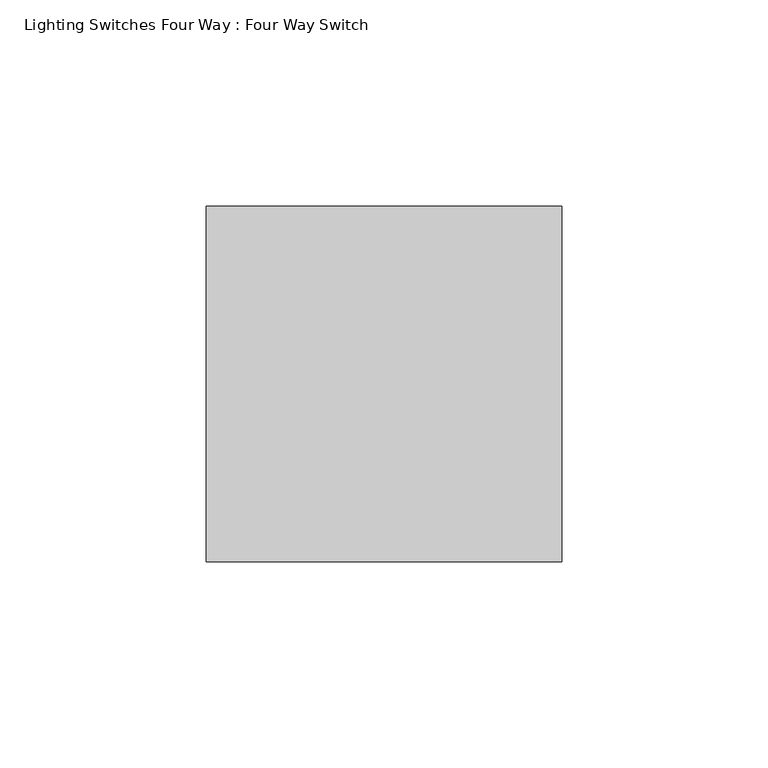
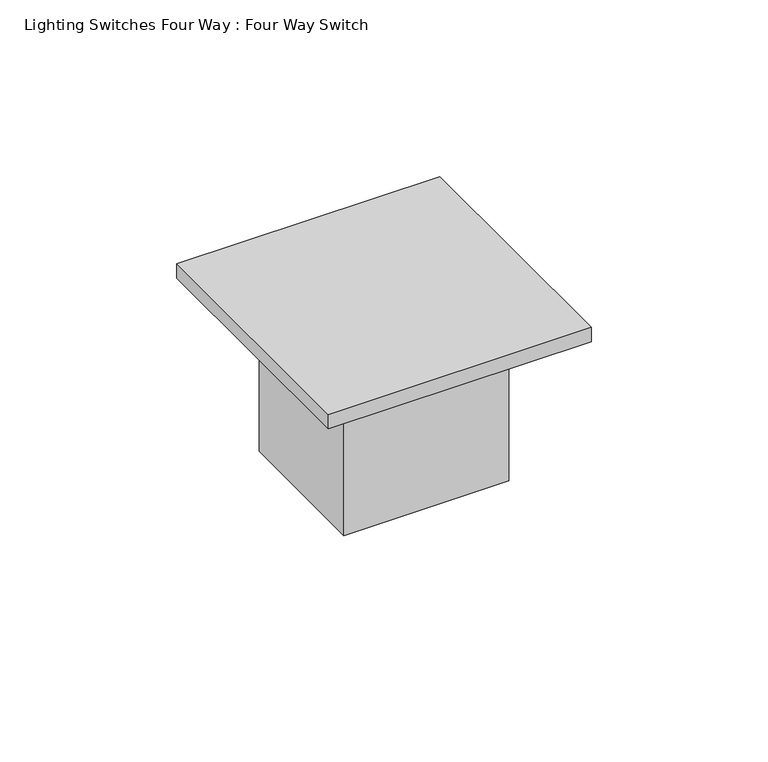
"""IFC4 building model written with IfcOpenShell, lengths in millimetres: switching device geometry, Lighting Switches Four Way : Four Way Switch."""

import ifcopenshell
import ifcopenshell.guid

model = None  # the IFC model being written
_history = None  # IfcOwnerHistory: only IFC2X3 demands one
_inside = {}  # id of a spatial element -> (the spatial element, [elements in it])
_under = {}  # id of a project, library or spatial element -> (it, [spatial elements below it])
_declared = {}  # id of a project -> (the project, [libraries it declares])
_typed = {}  # id of a type object -> (the type object, [elements of that type])
_made_of = {}  # id of a material, layer set ... -> (it, [elements and type objects made of it])


def new_model(schema):
    """Start an empty IFC model of exactly this schema.

    Asked for "IFC4X3", IfcOpenShell would pick the latest addendum, in which some entities
    have other attributes; the version numbers below select the first issue.
    IFC2X3 requires an IfcOwnerHistory on every rooted entity: one is made here for all.
    """
    global model, _history
    if schema == "IFC4X3":
        model = ifcopenshell.file(schema_version=(4, 3, 0, 0))
    else:
        model = ifcopenshell.file(schema=schema)
    _inside.clear()
    _under.clear()
    _declared.clear()
    _typed.clear()
    _made_of.clear()
    _history = None
    if model.schema == "IFC2X3":
        org = make("IfcOrganization", Name="unknown")
        user = make(
            "IfcPersonAndOrganization",
            ThePerson=make("IfcPerson", FamilyName="unknown"),
            TheOrganization=org,
        )
        app = make(
            "IfcApplication",
            ApplicationDeveloper=org,
            Version="unknown",
            ApplicationFullName="unknown",
            ApplicationIdentifier="unknown",
        )
        _history = make(
            "IfcOwnerHistory",
            OwningUser=user,
            OwningApplication=app,
            ChangeAction="ADDED",
            CreationDate=0,
        )
    return model


def make(cls, **values):
    """One entity of the class cls with the attributes given. An attribute that is None is left unset."""
    return model.create_entity(
        cls, **{name: value for name, value in values.items() if value is not None}
    )


def rooted(cls, **values):
    """An entity with a GlobalId (a new one), such as an element, a storey or a relation."""
    return make(cls, GlobalId=ifcopenshell.guid.new(), OwnerHistory=_history, **values)


def si_unit(unit_type, name, prefix=None):
    """IfcSIUnit, for example si_unit("LENGTHUNIT", "METRE", prefix="MILLI")."""
    return make("IfcSIUnit", UnitType=unit_type, Prefix=prefix, Name=name)


def assignment(units):
    """IfcUnitAssignment: the units of a project."""
    return None if units is None else make("IfcUnitAssignment", Units=units)


def point(xyz):
    """IfcCartesianPoint."""
    return None if xyz is None else make("IfcCartesianPoint", Coordinates=xyz)


def direction(xyz):
    """IfcDirection."""
    return None if xyz is None else make("IfcDirection", DirectionRatios=xyz)


def frame(location, z_axis=None, x_axis=None):
    """IfcAxis2Placement3D, a coordinate frame: its origin and axes. An axis left out is left unset."""
    return make(
        "IfcAxis2Placement3D",
        Location=point(location),
        Axis=direction(z_axis),
        RefDirection=direction(x_axis),
    )


def origin():
    """The frame at (0, 0, 0) with its axes left unset."""
    return frame((0.0, 0.0, 0.0))


def origin_with_axes():
    """The frame at (0, 0, 0) with the z axis (0, 0, 1) and the x axis (1, 0, 0) written out."""
    return frame((0.0, 0.0, 0.0), z_axis=(0.0, 0.0, 1.0), x_axis=(1.0, 0.0, 0.0))


def place(relative_to, where):
    """IfcLocalPlacement: puts the frame where relative to a parent placement (None: the world)."""
    return make(
        "IfcLocalPlacement", PlacementRelTo=relative_to, RelativePlacement=where
    )


def context(
    kind, dimensions, precision=None, world=None, true_north=None, identifier=None
):
    """IfcGeometricRepresentationContext, for example the 3D "Model" context."""
    return make(
        "IfcGeometricRepresentationContext",
        ContextIdentifier=identifier,
        ContextType=kind,
        CoordinateSpaceDimension=dimensions,
        Precision=precision,
        WorldCoordinateSystem=world,
        TrueNorth=true_north,
    )


def project(units=None, contexts=None):
    """IfcProject with its units and contexts."""
    return rooted(
        "IfcProject",
        Name="project",
        RepresentationContexts=contexts,
        UnitsInContext=assignment(units),
    )


def spatial(cls, under=None, at=None, **own):
    """A site, building, storey or space (cls), placed at a placement, below another one or the project."""
    s = rooted(cls, ObjectPlacement=at, **own)
    if under is not None:
        _under.setdefault(under.id(), (under, []))[1].append(s)
    return s


def polyline(points):
    """IfcPolyline through the points."""
    return make("IfcPolyline", Points=[point(p) for p in points])


def outline(outer, holes=None, kind="AREA"):
    """IfcArbitraryClosedProfileDef: a profile drawn as a closed curve; with holes, ...WithVoids."""
    if holes is None:
        return make("IfcArbitraryClosedProfileDef", ProfileType=kind, OuterCurve=outer)
    return make(
        "IfcArbitraryProfileDefWithVoids",
        ProfileType=kind,
        OuterCurve=outer,
        InnerCurves=holes,
    )


def extrude(swept, where, along, depth):
    """IfcExtrudedAreaSolid: the profile swept, set in the frame where, extruded along a direction by depth."""
    return make(
        "IfcExtrudedAreaSolid",
        SweptArea=swept,
        Position=where,
        ExtrudedDirection=direction(along),
        Depth=depth,
    )


def shape(context_of_items, identifier, shape_type, items):
    """IfcShapeRepresentation: the items that make up one representation, for example the "Body"."""
    return make(
        "IfcShapeRepresentation",
        ContextOfItems=context_of_items,
        RepresentationIdentifier=identifier,
        RepresentationType=shape_type,
        Items=items,
    )


def source(mapping_origin, context_of_items, identifier, shape_type, items):
    """IfcRepresentationMap: a shape defined once, which mapped items show again and again."""
    return make(
        "IfcRepresentationMap",
        MappingOrigin=mapping_origin,
        MappedRepresentation=shape(context_of_items, identifier, shape_type, items),
    )


def transform(
    local_origin,
    x_axis=None,
    y_axis=None,
    z_axis=None,
    scale=None,
    scale2=None,
    scale3=None,
    uniform=True,
):
    """IfcCartesianTransformationOperator3D, or its non-uniform kind. x_axis, y_axis, z_axis: its Axis1, 2, 3."""
    if uniform:
        return make(
            "IfcCartesianTransformationOperator3D",
            Axis1=direction(x_axis),
            Axis2=direction(y_axis),
            LocalOrigin=point(local_origin),
            Scale=scale,
            Axis3=direction(z_axis),
        )
    return make(
        "IfcCartesianTransformationOperator3DnonUniform",
        Axis1=direction(x_axis),
        Axis2=direction(y_axis),
        LocalOrigin=point(local_origin),
        Scale=scale,
        Axis3=direction(z_axis),
        Scale2=scale2,
        Scale3=scale3,
    )


def mapped(mapping_source, mapping_target):
    """IfcMappedItem: shows the shape of a source again, moved by a transform."""
    return make(
        "IfcMappedItem", MappingSource=mapping_source, MappingTarget=mapping_target
    )


def made_of(thing, what):
    """Note that an element or type object is made of a material, layer set ...; save() writes the relation."""
    if what is not None:
        _made_of.setdefault(what.id(), (what, []))[1].append(thing)
    return thing


def element(
    cls,
    number,
    at=None,
    inside=None,
    cuts=None,
    type_object=None,
    material=None,
    context=None,
    identifier="Body",
    shape_type=None,
    held_by="IfcProductDefinitionShape",
    body=None,
    shapes=None,
    **own,
):
    """One element of the class cls, such as IfcWall. Its Tag is "e" and its number.

    at: its placement. inside: the storey or other place that contains it. cuts: it is an
    opening in that element (IfcRelVoidsElement). A single representation is given by context,
    identifier, shape_type and body (its items); several are given by shapes. held_by: the class
    of the entity that holds the representations. save() writes the other relations.
    """
    e = rooted(cls, Tag="e%d" % number, ObjectPlacement=at, **own)
    if body is not None:
        shapes = [shape(context, identifier, shape_type, body)]
    if shapes is not None:
        e.Representation = make(held_by, Representations=shapes)
    if inside is not None:
        _inside.setdefault(inside.id(), (inside, []))[1].append(e)
    if cuts is not None:
        rooted(
            "IfcRelVoidsElement", RelatingBuildingElement=cuts, RelatedOpeningElement=e
        )
    if type_object is not None:
        _typed.setdefault(type_object.id(), (type_object, []))[1].append(e)
    return made_of(e, material)


def aggregate(whole, parts):
    """IfcRelAggregates: a whole, such as a stair, and the parts it consists of."""
    return rooted("IfcRelAggregates", RelatingObject=whole, RelatedObjects=parts)


def save(model, path):
    """Write the relations noted so far, then the file.

    IfcRelAggregates (storeys below a building ...), IfcRelContainedInSpatialStructure (elements
    in a storey), IfcRelDefinesByType, IfcRelAssociatesMaterial and IfcRelDeclares: one each for
    every whole, place, type object, material and project.
    """
    for whole, parts in _under.values():
        aggregate(whole, parts)
    for where, things in _inside.values():
        rooted(
            "IfcRelContainedInSpatialStructure",
            RelatedElements=things,
            RelatingStructure=where,
        )
    for kind, things in _typed.values():
        rooted("IfcRelDefinesByType", RelatedObjects=things, RelatingType=kind)
    for what, things in _made_of.values():
        rooted("IfcRelAssociatesMaterial", RelatedObjects=things, RelatingMaterial=what)
    for by, libraries in _declared.values():
        rooted("IfcRelDeclares", RelatingContext=by, RelatedDefinitions=libraries)
    model.write(path)


def lighting_switches_four_way_four_way_switch_ab144c04(model_context):
    return source(origin(), model_context, "Body", "SweptSolid", [
        extrude(outline(polyline([(43.0, -86.0), (-43.0, -86.0), (-43.0, 0.0), (43.0, 0.0), (43.0, -86.0)])), origin_with_axes(), (0.0, 0.0, 1.0), 5.0),
        extrude(outline(polyline([(27.0, -67.0), (-27.0, -67.0), (-27.0, -19.0), (27.0, -19.0), (27.0, -67.0)])), frame((0.0, 0.0, -54.0), z_axis=(0.0, 0.0, 1.0), x_axis=(1.0, 0.0, 0.0)), (0.0, 0.0, 1.0), 54.0),
    ])


if __name__ == "__main__":
    model = new_model("IFC4")
    model_context = context("Model", 3, world=origin())
    ifc_project = project(units=[si_unit("LENGTHUNIT", "METRE", prefix="MILLI")], contexts=[model_context])
    site = spatial("IfcSite", under=ifc_project)
    building = spatial("IfcBuilding", under=site)
    placement = place(None, origin())
    lighting_switches_four_way_four_way_switch_shape = lighting_switches_four_way_four_way_switch_ab144c04(model_context)
    element("IfcSwitchingDevice", 1, ObjectType="Lighting Switches Four Way : Four Way Switch", at=placement, inside=building, context=model_context, shape_type="MappedRepresentation", body=[
        mapped(lighting_switches_four_way_four_way_switch_shape, transform((0.0, 0.0, 0.0), x_axis=(1.0, 0.0, 0.0), y_axis=(0.0, 1.0, 0.0), z_axis=(0.0, 0.0, 1.0))),
    ])
    save(model, "model.ifc")

# Revit data of these elements
# Type "Lighting Switches Four Way : Four Way Switch"
#   Type Mark = "Lighting Switches Four Way"
#   Classification.OmniClass.21.Number = "21-04 50 40 10"
#   Classification.OmniClass.21.Description = "Lighting Control"
#   Classification.UniFormat.II.Description = "Lighting Control"
#   Classification.OmniClass.23.Number = "23-35 37 00"
#   Classification.OmniClass.23.Description = "Electrical Switches"
#   Classification.UniFormat.II.Number = "D5040.10"
#   COBie.Type.CreatedBy = "info@mma.ie"
#   COBie.Type.CreatedOn = "2017-07-25T10:15:16"
#   COBie.Type.Name = "Lighting Switches Four Way"
#   COBie.Type.Category = "23-35 37 00 : Electrical Switches"
#   COBie.Type.Description = "Lighting Switches Four Way_Four Way Switch"
#   COBie.Type.AssetType = "Fixed"
#   COBie.Type.Manufacturer = ""
#   COBie.Type.ModelNumber = ""
#   Label = "4"
#   Keynote = "26 36 13.D"
#   COBie.Type.ReplacementCost = 0
#   Switch Voltage [instance default] = 230 V
#   Default Elevation = 1200 mm
#   Apparent Load = 0 VA
#   4.W.S. Width = 86 mm
#   4.W.S. Height = 86 mm
#   4.W.S. Depth = 59 mm
#   COBie.Type = yes
#   Visibility 7 = no
#   Visibility 6 = no
#   Visibility 5 = no
#   Visibility 4 = yes
#   Visibility 3 = no
#   Visibility 2 = no
#   Visibility 1 = no
#   Ballast Number of Poles = 1
#   Load Classification = Other
#   4.W.S. Material = Metal - Chrome
# Materials
#   "Metal - Chrome": class "Metal", colour RGB 17 17 17, transparency 0, Comments = "Rendering appearance not upgraded "
